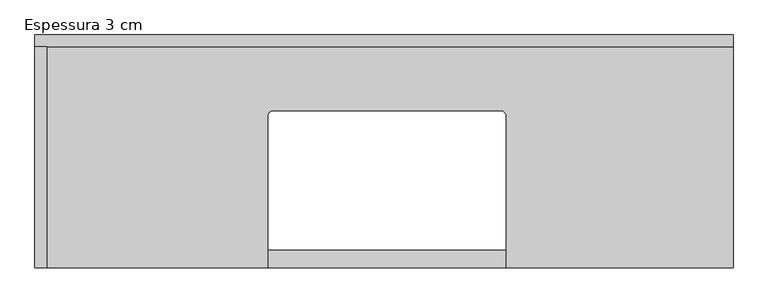
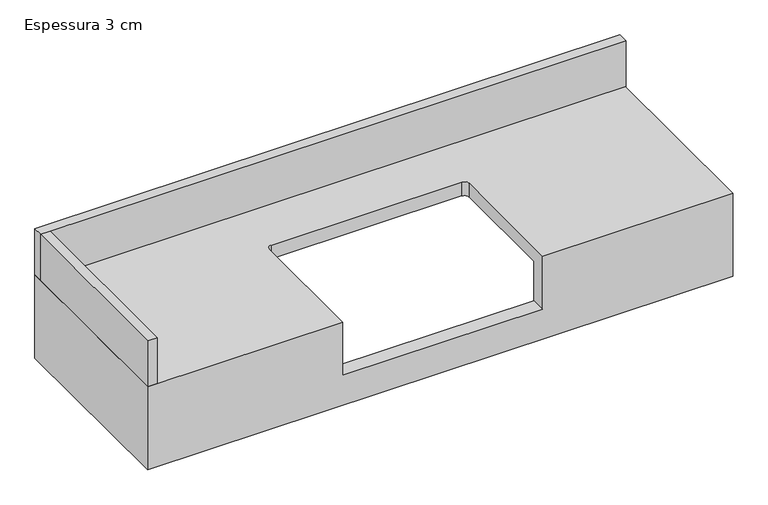
"""IFC4 building model written with IfcOpenShell, lengths in millimetres: furniture geometry, CC_BANCADA BANHEIRO COM CUBA_CANTO RETO : Espessura 3 cm."""

from ifc_helpers import new_model, si_unit, frame, origin, place, context, project, spatial, polyline, circle_curve, outline, extrude, source, transform, mapped, element, save
from ifc_brep_helpers import plane_surface, revolved_surface, advanced_brep


def espessura_3_cm_a8edac31(model_context):
    return source(origin(), model_context, "Body", "SolidModel", [
        advanced_brep(
        [(750.0, 300.0, 860.0), (-450.0, 300.0, 860.0), (-450.0, -100.0, 860.0), (-50.0, -100.0, 860.0), (-50.0, 160.0, 860.0), (-40.0, 170.0, 860.0), (350.0, 170.0, 860.0), (360.0, 160.0, 860.0), (360.0, -100.0, 860.0), (750.0, -100.0, 860.0), (750.0, 300.0, 680.0), (720.0, 300.0, 680.0), (720.0, 300.0, 830.0), (-420.0, 300.0, 830.0), (-420.0, 300.0, 680.0), (-450.0, 300.0, 680.0), (-450.0, -100.0, 680.0), (750.0, -100.0, 680.0), (360.0, -100.0, 745.0), (-50.0, -100.0, 745.0), (720.0, -70.0, 830.0), (360.0, -70.0, 830.0), (360.0, 160.0, 830.0), (350.0, 170.0, 830.0), (-40.0, 170.0, 830.0), (-50.0, 160.0, 830.0), (-50.0, -70.0, 830.0), (-420.0, -70.0, 830.0), (-420.0, -70.0, 680.0), (-50.0, -70.0, 745.0), (360.0, -70.0, 745.0), (720.0, -70.0, 680.0)],
        [
            (0, 1),
            (1, 2),
            (2, 3),
            (3, 4),
            (4, 5, circle_curve(frame((-40.0, 160.0, 860.0), z_axis=(0.0, 0.0, -1.0), x_axis=(0.0, 1.0, 0.0)), 10.0)),
            (5, 6),
            (6, 7, circle_curve(frame((350.0, 160.0, 860.0), z_axis=(0.0, 0.0, -1.0), x_axis=(0.0, 1.0, 0.0)), 10.0)),
            (7, 8),
            (8, 9),
            (9, 0),
            (0, 10),
            (10, 11),
            (11, 12),
            (12, 13),
            (13, 14),
            (14, 15),
            (15, 1),
            (15, 16),
            (16, 2),
            (16, 17),
            (17, 9),
            (8, 18),
            (18, 19),
            (19, 3),
            (17, 10),
            (12, 20),
            (20, 21),
            (21, 22),
            (22, 23, circle_curve(frame((350.0, 160.0, 830.0), z_axis=(0.0, 0.0, 1.0), x_axis=(0.0, 1.0, 0.0)), 10.0)),
            (23, 24),
            (24, 25, circle_curve(frame((-40.0, 160.0, 830.0), z_axis=(0.0, 0.0, 1.0), x_axis=(0.0, 1.0, 0.0)), 10.0)),
            (25, 26),
            (26, 27),
            (27, 13),
            (27, 28),
            (28, 14),
            (26, 29),
            (29, 30),
            (30, 21),
            (20, 31),
            (31, 28),
            (11, 31),
            (5, 24),
            (23, 6),
            (18, 30),
            (29, 19),
            (4, 25),
            (7, 22),
        ],
        [
            plane_surface(frame((-450.0, 300.0, 860.0), z_axis=(0.0, 0.0, 1.0), x_axis=(-1.0, 0.0, 0.0))),
            plane_surface(frame((750.0, 300.0, 860.0), z_axis=(0.0, 1.0, 0.0), x_axis=(0.0, 0.0, -1.0))),
            plane_surface(frame((-450.0, 300.0, 860.0), z_axis=(-1.0, 0.0, 0.0), x_axis=(0.0, 0.0, -1.0))),
            plane_surface(frame((-450.0, -100.0, 860.0), z_axis=(0.0, -1.0, 0.0), x_axis=(0.0, 0.0, -1.0))),
            plane_surface(frame((750.0, -100.0, 860.0), z_axis=(1.0, 0.0, 0.0), x_axis=(0.0, 0.0, -1.0))),
            plane_surface(frame((-420.0, 300.0, 830.0), z_axis=(0.0, 0.0, -1.0), x_axis=(-1.0, 0.0, 0.0))),
            plane_surface(frame((-420.0, 300.0, 830.0), z_axis=(1.0, 0.0, 0.0), x_axis=(0.0, 0.0, -1.0))),
            plane_surface(frame((-420.0, -70.0, 830.0), z_axis=(0.0, 1.0, 0.0), x_axis=(0.0, 0.0, -1.0))),
            plane_surface(frame((720.0, -70.0, 830.0), z_axis=(-1.0, 0.0, 0.0), x_axis=(0.0, 0.0, -1.0))),
            plane_surface(frame((750.0, -100.0, 680.0), z_axis=(0.0, 0.0, -1.0), x_axis=(0.0, 1.0, 0.0))),
            plane_surface(frame((-40.0, 170.0, 745.0), z_axis=(0.0, -1.0, 0.0), x_axis=(0.0, 0.0, 1.0))),
            plane_surface(frame((350.0, 170.0, 745.0), z_axis=(0.0, 0.0, 1.0), x_axis=(1.0, 0.0, 0.0))),
            revolved_surface(polyline([(-40.0, 170.0, 830.0), (-40.0, 170.0, 860.0)]), (-40.0, 160.0, 900.0), (0.0, 0.0, -1.0)),
            plane_surface(frame((-50.0, -230.0, 745.0), z_axis=(1.0, 0.0, 0.0), x_axis=(0.0, 0.0, 1.0))),
            plane_surface(frame((360.0, 160.0, 745.0), z_axis=(-1.0, 0.0, 0.0), x_axis=(0.0, 0.0, 1.0))),
            revolved_surface(polyline([(350.0, 170.0, 830.0), (350.0, 170.0, 860.0)]), (350.0, 160.0, 900.0), (0.0, 0.0, -1.0)),
        ],
        [
            (0, [[1, 2, 3, 4, 5, 6, 7, 8, 9, 10]]),
            (1, [[-1, 11, 12, 13, 14, 15, 16, 17]]),
            (2, [[-2, -17, 18, 19]]),
            (3, [[-3, -19, 20, 21, -9, 22, 23, 24]]),
            (4, [[-10, -21, 25, -11]]),
            (5, [[26, 27, 28, 29, 30, 31, 32, 33, 34, -14]]),
            (6, [[-34, 35, 36, -15]]),
            (7, [[-33, 37, 38, 39, -27, 40, 41, -35]]),
            (8, [[-26, -13, 42, -40]]),
            (9, [[-12, -25, -20, -18, -16, -36, -41, -42]]),
            (10, [[-6, 43, -30, 44]]),
            (11, [[-23, 45, -38, 46]]),
            (12, [[-5, 47, -31, -43]]),
            (13, [[-4, -24, -46, -37, -32, -47]]),
            (14, [[-8, 48, -28, -39, -45, -22]]),
            (15, [[-7, -44, -29, -48]]),
        ],
    ),
        extrude(outline(polyline([(-430.0, -100.0), (-450.0, -100.0), (-450.0, 280.0), (-430.0, 280.0), (-430.0, -100.0)])), frame((0.0, 0.0, 860.0), z_axis=(0.0, 0.0, 1.0), x_axis=(1.0, 0.0, 0.0)), (0.0, 0.0, 1.0), 100.0),
        extrude(outline(polyline([(750.0, 300.0), (750.0, 280.0), (-450.0, 280.0), (-450.0, 300.0), (750.0, 300.0)])), frame((0.0, 0.0, 860.0), z_axis=(0.0, 0.0, 1.0), x_axis=(1.0, 0.0, 0.0)), (0.0, 0.0, 1.0), 100.0),
    ])


if __name__ == "__main__":
    model = new_model("IFC4")
    model_context = context("Model", 3, world=origin())
    ifc_project = project(units=[si_unit("LENGTHUNIT", "METRE", prefix="MILLI")], contexts=[model_context])
    site = spatial("IfcSite", under=ifc_project)
    building = spatial("IfcBuilding", under=site)
    placement = place(None, origin())
    espessura_3_cm_shape = espessura_3_cm_a8edac31(model_context)
    element("IfcFurniture", 1, ObjectType="CC_BANCADA BANHEIRO COM CUBA_CANTO RETO : Espessura 3 cm", at=placement, inside=building, context=model_context, shape_type="MappedRepresentation", body=[
        mapped(espessura_3_cm_shape, transform((0.0, 0.0, 0.0), x_axis=(1.0, 0.0, 0.0), y_axis=(0.0, 1.0, 0.0), z_axis=(0.0, 0.0, 1.0))),
    ])
    save(model, "model.ifc")

# Revit data of these elements
# Type "CC_BANCADA BANHEIRO COM CUBA_CANTO RETO : Espessura 3 cm"
#   Uso HS [instance default] = ""
#   h TESTEIRA AUX [instance default] = 0.15 m
#   Altura testeira [instance default] = 0.15 m
#   Altura rodapia [instance default] = 0.10 m
#   Espessura rodapia [instance default] = 0.02 m
#   Prof/2 [instance default] = 0.20 m
#   Offset cuba esquerda [instance default] = 0.40 m
#   Depth [instance default] = 1.20 m
#   Width [instance default] = 0.40 m
#   Espessura bancada = 0.03 m
#   Comprimento [instance default] = 1.20 m
#   Height [instance default] = 0.86 m
#   Testeira [instance default] = yes
#   Rodapia fundo [instance default] = no
#   Rodapia esquerda [instance default] = no
#   Rodapia direita [instance default] = no
#   Material porta-toalha [instance default] = .CROMADO
#   Material hidráulico [instance default] = .CROMADO
#   Material cuba [instance default] = .PORCELANA BRANCA
#   Material bancada [instance default] = .GRANITO_BRANCO_ITAUNAS
#   Assembly Code = ""
# Element 1 (IfcFurniture, "CC_BANCADA BANHEIRO COM CUBA_CANTO RETO : Espessura 3 cm")
#   Uso HS = "BANHO SUÍTE 2"
#   Rodapia fundo = yes
#   Rodapia esquerda = yes
#   Materials on its faces: ".GRANITO_BRANCO_ITAUNAS"
# Materials
#   ".CROMADO": class "CC_METAIS", colour RGB 211 223 226, transparency 0, Cost = 0
#   ".PORCELANA BRANCA": class "CC_PORCELANA", colour RGB 230 230 230, transparency 0, Cost = 0
#   ".GRANITO_BRANCO_ITAUNAS": class ".CC_PEDRA REVEST.", colour RGB 202 195 174, transparency 0, Description = "Revestimento em granito", Cost = 0
